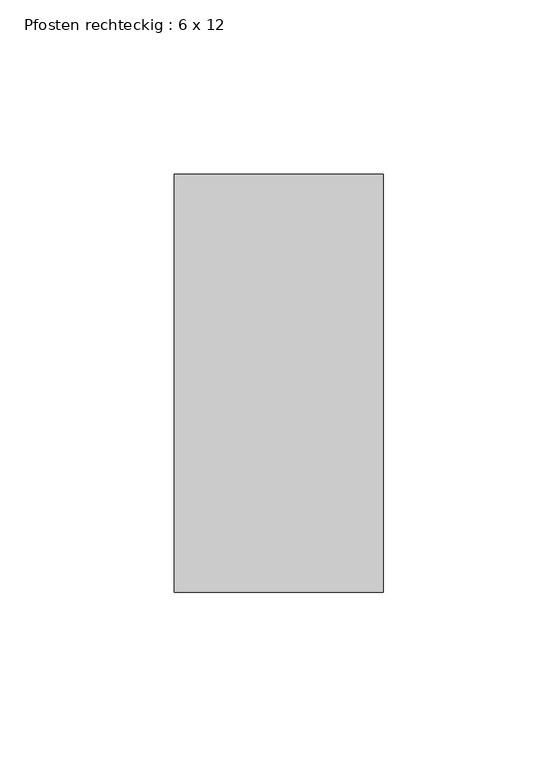
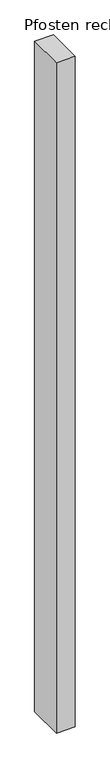
"""IFC4 building model written with IfcOpenShell, lengths in millimetres: member geometry, Pfosten rechteckig : 6 x 12."""

from ifc_helpers import new_model, si_unit, frame, origin, place, context, project, spatial, polyline, outline, extrude, source, transform, mapped, element, save


def pfosten_rechteckig_6_x_12_b3245d14(model_context):
    return source(origin(), model_context, "Body", "SweptSolid", [
        extrude(outline(polyline([(0.0, 60.0), (0.0, -60.0), (-60.0, -60.0), (-60.0, 60.0), (0.0, 60.0)])), frame((0.0, 0.0, -2264.8398838), z_axis=(0.0, 0.0, 1.0), x_axis=(1.0, 0.0, 0.0)), (0.0, 0.0, 1.0), 2264.8398838),
    ])


if __name__ == "__main__":
    model = new_model("IFC4")
    model_context = context("Model", 3, world=origin())
    ifc_project = project(units=[si_unit("LENGTHUNIT", "METRE", prefix="MILLI")], contexts=[model_context])
    site = spatial("IfcSite", under=ifc_project)
    building = spatial("IfcBuilding", under=site)
    placement = place(None, origin())
    pfosten_rechteckig_6_x_12_shape = pfosten_rechteckig_6_x_12_b3245d14(model_context)
    element("IfcMember", 1, ObjectType="Pfosten rechteckig : 6 x 12", at=placement, inside=building, context=model_context, shape_type="MappedRepresentation", body=[
        mapped(pfosten_rechteckig_6_x_12_shape, transform((0.0, 0.0, 0.0), x_axis=(1.0, 0.0, 0.0), y_axis=(0.0, 1.0, 0.0), z_axis=(0.0, 0.0, 1.0))),
    ])
    save(model, "model.ifc")

# Revit data of these elements
# Type "Pfosten rechteckig : 6 x 12"
#   built-in parameter 1007304 = 0.393701 (stored number, unit not read)
#   built-in parameter 1007301 = 0.0984252 (stored number, unit not read)
#   built-in parameter 1007300 = 0.0984252 (stored number, unit not read)
# Element 1 (IfcMember, "Pfosten rechteckig : 6 x 12")
#   Materials on its faces: "Metall - verzinkt"
# Materials
#   "Metall - verzinkt": class "Allgemeines", colour RGB 200 200 200, transparency 0, Cost = 0
